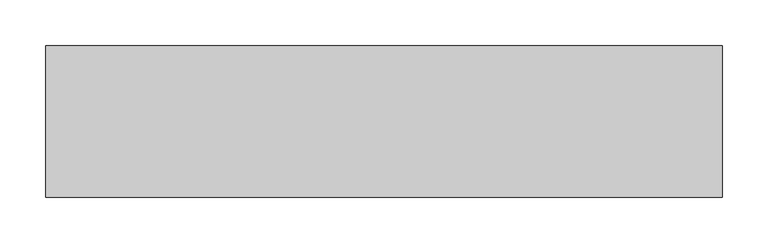
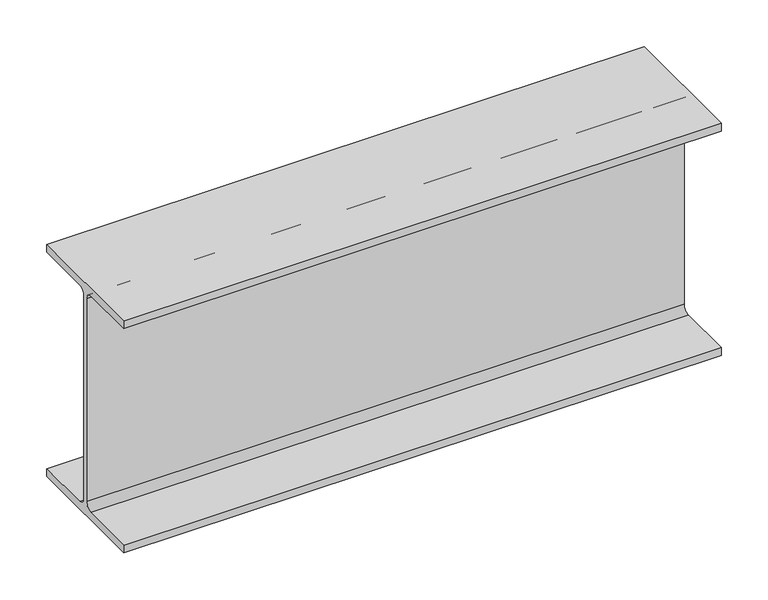
"""IFC4 building model written with IfcOpenShell, lengths in millimetres: beam geometry, Old_Steel Beam_H-KSD3502 : H_SB_ASB_H-300×300x10x15."""

from ifc_helpers import new_model, si_unit, point, frame, frame_2d, origin, place, context, project, spatial, polyline, circle_curve, trimmed, segment, composite_curve, outline, extrude, source, transform, mapped, element, save


def beam_5dfb366b(model_context):
    return source(origin(), model_context, "Body", "SweptSolid", [
        extrude(outline(composite_curve([segment(polyline([(82.5, -141.5), (82.5, -151.7), (-82.5, -151.7), (-82.5, -141.5), (-11.9, -141.5)]), True, "CONTINUOUS"), segment(trimmed(circle_curve(frame_2d((-11.9, -132.6)), 8.9), [point((-11.9, -141.5))], [point((-3.0, -132.6))], True, "CARTESIAN"), True, "CONTINUOUS"), segment(polyline([(-3.0, -132.6), (-3.0, 132.6)]), True, "CONTINUOUS"), segment(trimmed(circle_curve(frame_2d((-11.9, 132.6)), 8.9), [point((-3.0, 132.6))], [point((-11.9, 141.5))], True, "CARTESIAN"), True, "CONTINUOUS"), segment(polyline([(-11.9, 141.5), (-82.5, 141.5), (-82.5, 151.7), (82.5, 151.7), (82.5, 141.5), (11.9, 141.5)]), True, "CONTINUOUS"), segment(trimmed(circle_curve(frame_2d((11.9, 132.6)), 8.9), [point((11.9, 141.5))], [point((3.0, 132.6))], True, "CARTESIAN"), True, "CONTINUOUS"), segment(polyline([(3.0, 132.6), (3.0, -132.6)]), True, "CONTINUOUS"), segment(trimmed(circle_curve(frame_2d((11.9, -132.6)), 8.9), [point((3.0, -132.6))], [point((11.9, -141.5))], True, "CARTESIAN"), True, "CONTINUOUS"), segment(polyline([(11.9, -141.5), (82.5, -141.5)]), True, "CONTINUOUS")], self_intersect=False)), frame((-502.5, 0.0, 0.0), z_axis=(1.0, 0.0, 0.0), x_axis=(0.0, 1.0, 0.0)), (0.0, 0.0, 1.0), 738.1129602),
    ])


if __name__ == "__main__":
    model = new_model("IFC4")
    model_context = context("Model", 3, world=origin())
    ifc_project = project(units=[si_unit("LENGTHUNIT", "METRE", prefix="MILLI")], contexts=[model_context])
    site = spatial("IfcSite", under=ifc_project)
    building = spatial("IfcBuilding", under=site)
    placement = place(None, origin())
    beam_shape = beam_5dfb366b(model_context)
    element("IfcBeam", 1, ObjectType="Old_Steel Beam_H-KSD3502 : H_SB_ASB_H-300×300x10x15", at=placement, inside=building, context=model_context, shape_type="MappedRepresentation", body=[
        mapped(beam_shape, transform((0.0, 0.0, 0.0), x_axis=(1.0, 0.0, 0.0), y_axis=(0.0, 1.0, 0.0), z_axis=(0.0, 0.0, 1.0))),
    ])
    save(model, "model.ifc")

# Revit data of these elements
# Type "Old_Steel Beam_H-KSD3502 : H_SB_ASB_H-300×300x10x15"
#   Width = 30.0 cm
#   Web Thickness = 1.0 cm
#   Web Fillet = 1.8 cm
#   Warping Constant = 1370670.0 cm⁶
#   Torsional Moment of Inertia = 77.00 cm⁴
#   Torsional Modulus = 1.0 cm³
#   Section Area = 119.8 cm²
#   Plastic Modulus weak axis = 684.0 cm³
#   Plastic Modulus strong axis = 1500.0 cm³
#   Perimeter = 1.75 m²/m
#   Nominal Weight = 94.00 kgf/m
#   Moment of Inertia weak axis = 6750.00 cm⁴
#   Moment of Inertia strong axis = 20400.00 cm⁴
#   Height = 30.0 cm
#   Flange Thickness = 1.5 cm
#   Elastic Modulus weak axis = 450.0 cm³
#   Elastic Modulus strong axis = 1360.0 cm³
#   Centroid Vertical = 15.0 cm
#   Centroid Horizontal = 15.0 cm
#   Length [instance default] = 1.5240 m
#   Structural Material [instance default] = Steel, 45-345
#   Assembly Code = ""
# Element 1 (IfcBeam, "Old_Steel Beam_H-KSD3502 : H_SB_ASB_H-300×300x10x15")
#   Structural Material = none
# Materials
#   "Steel, 45-345": class "Metal", colour RGB 189 187 185, transparency 0, Description = "Steel 345 MPa", Cost = 0
